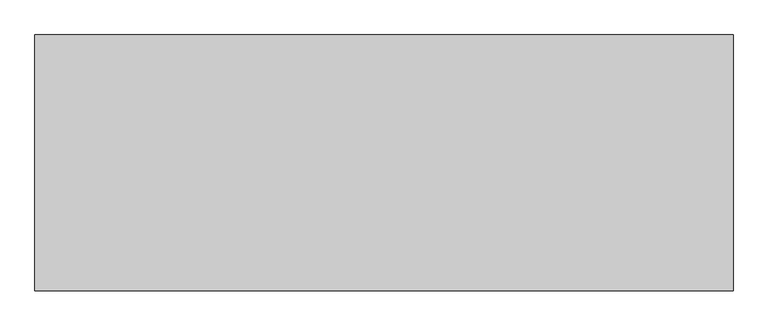
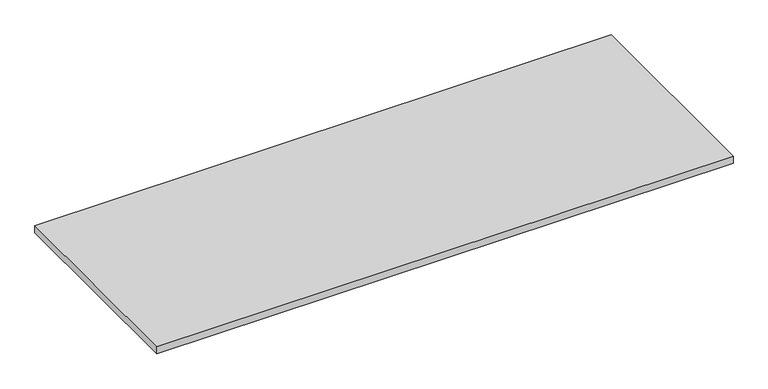
"""IFC4 building model written with IfcOpenShell, lengths in millimetres: proxy geometry, Plywood025 1374 : Plywood025 1374."""

from ifc_helpers import new_model, si_unit, frame, origin, place, context, project, spatial, polyline, outline, extrude, source, transform, mapped, element, save


def generic_models_cbdf57ab(model_context):
    return source(origin(), model_context, "Body", "SweptSolid", [
        extrude(outline(polyline([(3694.2883192, 8857.2125834), (3694.2883192, 9590.6375834), (5694.2883192, 9590.6375834), (5694.2883192, 8857.2125834), (3694.2883192, 8857.2125834)])), frame((0.0, 0.0, 36531.296), z_axis=(0.0, 0.0, 1.0), x_axis=(1.0, 0.0, 0.0)), (0.0, 0.0, 1.0), 25.4),
    ])


if __name__ == "__main__":
    model = new_model("IFC4")
    model_context = context("Model", 3, world=origin())
    ifc_project = project(units=[si_unit("LENGTHUNIT", "METRE", prefix="MILLI")], contexts=[model_context])
    site = spatial("IfcSite", under=ifc_project)
    building = spatial("IfcBuilding", under=site)
    placement = place(None, origin())
    generic_models_shape = generic_models_cbdf57ab(model_context)
    element("IfcBuildingElementProxy", 1, Name="Plywood025 1374 : Plywood025 1374", ObjectType="Plywood025 1374 : Plywood025 1374", at=placement, inside=building, context=model_context, shape_type="MappedRepresentation", body=[
        mapped(generic_models_shape, transform((0.0, 0.0, 0.0), x_axis=(1.0, 0.0, 0.0), y_axis=(0.0, 1.0, 0.0), z_axis=(0.0, 0.0, 1.0))),
    ])
    save(model, "model.ifc")

# Revit data of these elements
# Type "Plywood025 1374 : Plywood025 1374"
#   NameOverride = "Plywood025"
# Element 1 (IfcBuildingElementProxy, "Plywood025 1374 : Plywood025 1374")
#   Materials on its faces: "3/4\" TREATED CDX PLYWOOD OVER 6 MIL POLYETHYLENE VAPOR BARRIER"
# Materials
#   "3/4\" TREATED CDX PLYWOOD OVER 6 MIL POLYETHYLENE VAPOR BARRIER": class "Unassigned", colour RGB 67 103 56, transparency 0, Cost = 0
